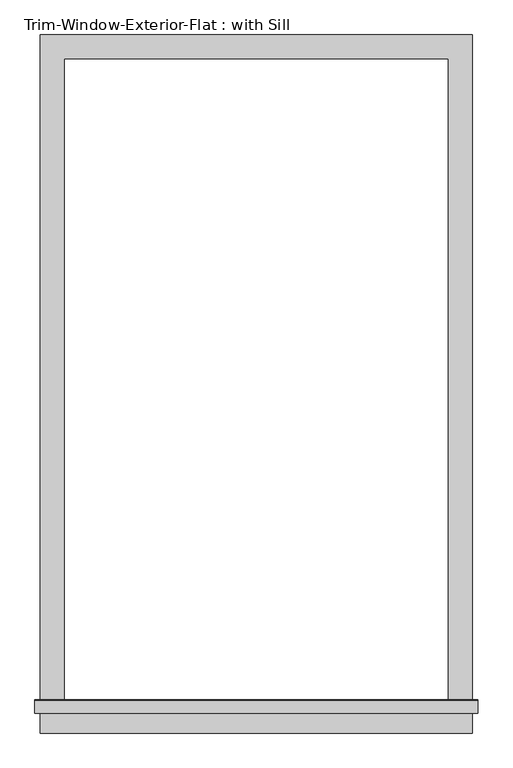
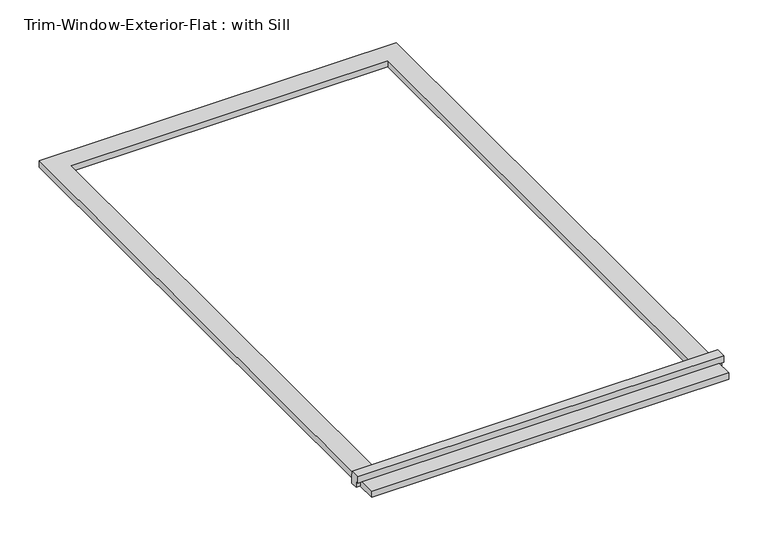
"""IFC4 building model written with IfcOpenShell, lengths in millimetres: proxy geometry, Trim-Window-Exterior-Flat : with Sill."""

import ifcopenshell
import ifcopenshell.guid

model = None  # the IFC model being written
_history = None  # IfcOwnerHistory: only IFC2X3 demands one
_inside = {}  # id of a spatial element -> (the spatial element, [elements in it])
_under = {}  # id of a project, library or spatial element -> (it, [spatial elements below it])
_declared = {}  # id of a project -> (the project, [libraries it declares])
_typed = {}  # id of a type object -> (the type object, [elements of that type])
_made_of = {}  # id of a material, layer set ... -> (it, [elements and type objects made of it])


def new_model(schema):
    """Start an empty IFC model of exactly this schema.

    Asked for "IFC4X3", IfcOpenShell would pick the latest addendum, in which some entities
    have other attributes; the version numbers below select the first issue.
    IFC2X3 requires an IfcOwnerHistory on every rooted entity: one is made here for all.
    """
    global model, _history
    if schema == "IFC4X3":
        model = ifcopenshell.file(schema_version=(4, 3, 0, 0))
    else:
        model = ifcopenshell.file(schema=schema)
    _inside.clear()
    _under.clear()
    _declared.clear()
    _typed.clear()
    _made_of.clear()
    _history = None
    if model.schema == "IFC2X3":
        org = make("IfcOrganization", Name="unknown")
        user = make(
            "IfcPersonAndOrganization",
            ThePerson=make("IfcPerson", FamilyName="unknown"),
            TheOrganization=org,
        )
        app = make(
            "IfcApplication",
            ApplicationDeveloper=org,
            Version="unknown",
            ApplicationFullName="unknown",
            ApplicationIdentifier="unknown",
        )
        _history = make(
            "IfcOwnerHistory",
            OwningUser=user,
            OwningApplication=app,
            ChangeAction="ADDED",
            CreationDate=0,
        )
    return model


def make(cls, **values):
    """One entity of the class cls with the attributes given. An attribute that is None is left unset."""
    return model.create_entity(
        cls, **{name: value for name, value in values.items() if value is not None}
    )


def rooted(cls, **values):
    """An entity with a GlobalId (a new one), such as an element, a storey or a relation."""
    return make(cls, GlobalId=ifcopenshell.guid.new(), OwnerHistory=_history, **values)


def si_unit(unit_type, name, prefix=None):
    """IfcSIUnit, for example si_unit("LENGTHUNIT", "METRE", prefix="MILLI")."""
    return make("IfcSIUnit", UnitType=unit_type, Prefix=prefix, Name=name)


def assignment(units):
    """IfcUnitAssignment: the units of a project."""
    return None if units is None else make("IfcUnitAssignment", Units=units)


def point(xyz):
    """IfcCartesianPoint."""
    return None if xyz is None else make("IfcCartesianPoint", Coordinates=xyz)


def direction(xyz):
    """IfcDirection."""
    return None if xyz is None else make("IfcDirection", DirectionRatios=xyz)


def frame(location, z_axis=None, x_axis=None):
    """IfcAxis2Placement3D, a coordinate frame: its origin and axes. An axis left out is left unset."""
    return make(
        "IfcAxis2Placement3D",
        Location=point(location),
        Axis=direction(z_axis),
        RefDirection=direction(x_axis),
    )


def origin():
    """The frame at (0, 0, 0) with its axes left unset."""
    return frame((0.0, 0.0, 0.0))


def origin_with_axes():
    """The frame at (0, 0, 0) with the z axis (0, 0, 1) and the x axis (1, 0, 0) written out."""
    return frame((0.0, 0.0, 0.0), z_axis=(0.0, 0.0, 1.0), x_axis=(1.0, 0.0, 0.0))


def place(relative_to, where):
    """IfcLocalPlacement: puts the frame where relative to a parent placement (None: the world)."""
    return make(
        "IfcLocalPlacement", PlacementRelTo=relative_to, RelativePlacement=where
    )


def context(
    kind, dimensions, precision=None, world=None, true_north=None, identifier=None
):
    """IfcGeometricRepresentationContext, for example the 3D "Model" context."""
    return make(
        "IfcGeometricRepresentationContext",
        ContextIdentifier=identifier,
        ContextType=kind,
        CoordinateSpaceDimension=dimensions,
        Precision=precision,
        WorldCoordinateSystem=world,
        TrueNorth=true_north,
    )


def project(units=None, contexts=None):
    """IfcProject with its units and contexts."""
    return rooted(
        "IfcProject",
        Name="project",
        RepresentationContexts=contexts,
        UnitsInContext=assignment(units),
    )


def spatial(cls, under=None, at=None, **own):
    """A site, building, storey or space (cls), placed at a placement, below another one or the project."""
    s = rooted(cls, ObjectPlacement=at, **own)
    if under is not None:
        _under.setdefault(under.id(), (under, []))[1].append(s)
    return s


def polyline(points):
    """IfcPolyline through the points."""
    return make("IfcPolyline", Points=[point(p) for p in points])


def outline(outer, holes=None, kind="AREA"):
    """IfcArbitraryClosedProfileDef: a profile drawn as a closed curve; with holes, ...WithVoids."""
    if holes is None:
        return make("IfcArbitraryClosedProfileDef", ProfileType=kind, OuterCurve=outer)
    return make(
        "IfcArbitraryProfileDefWithVoids",
        ProfileType=kind,
        OuterCurve=outer,
        InnerCurves=holes,
    )


def extrude(swept, where, along, depth):
    """IfcExtrudedAreaSolid: the profile swept, set in the frame where, extruded along a direction by depth."""
    return make(
        "IfcExtrudedAreaSolid",
        SweptArea=swept,
        Position=where,
        ExtrudedDirection=direction(along),
        Depth=depth,
    )


def shape(context_of_items, identifier, shape_type, items):
    """IfcShapeRepresentation: the items that make up one representation, for example the "Body"."""
    return make(
        "IfcShapeRepresentation",
        ContextOfItems=context_of_items,
        RepresentationIdentifier=identifier,
        RepresentationType=shape_type,
        Items=items,
    )


def source(mapping_origin, context_of_items, identifier, shape_type, items):
    """IfcRepresentationMap: a shape defined once, which mapped items show again and again."""
    return make(
        "IfcRepresentationMap",
        MappingOrigin=mapping_origin,
        MappedRepresentation=shape(context_of_items, identifier, shape_type, items),
    )


def transform(
    local_origin,
    x_axis=None,
    y_axis=None,
    z_axis=None,
    scale=None,
    scale2=None,
    scale3=None,
    uniform=True,
):
    """IfcCartesianTransformationOperator3D, or its non-uniform kind. x_axis, y_axis, z_axis: its Axis1, 2, 3."""
    if uniform:
        return make(
            "IfcCartesianTransformationOperator3D",
            Axis1=direction(x_axis),
            Axis2=direction(y_axis),
            LocalOrigin=point(local_origin),
            Scale=scale,
            Axis3=direction(z_axis),
        )
    return make(
        "IfcCartesianTransformationOperator3DnonUniform",
        Axis1=direction(x_axis),
        Axis2=direction(y_axis),
        LocalOrigin=point(local_origin),
        Scale=scale,
        Axis3=direction(z_axis),
        Scale2=scale2,
        Scale3=scale3,
    )


def mapped(mapping_source, mapping_target):
    """IfcMappedItem: shows the shape of a source again, moved by a transform."""
    return make(
        "IfcMappedItem", MappingSource=mapping_source, MappingTarget=mapping_target
    )


def made_of(thing, what):
    """Note that an element or type object is made of a material, layer set ...; save() writes the relation."""
    if what is not None:
        _made_of.setdefault(what.id(), (what, []))[1].append(thing)
    return thing


def element(
    cls,
    number,
    at=None,
    inside=None,
    cuts=None,
    type_object=None,
    material=None,
    context=None,
    identifier="Body",
    shape_type=None,
    held_by="IfcProductDefinitionShape",
    body=None,
    shapes=None,
    **own,
):
    """One element of the class cls, such as IfcWall. Its Tag is "e" and its number.

    at: its placement. inside: the storey or other place that contains it. cuts: it is an
    opening in that element (IfcRelVoidsElement). A single representation is given by context,
    identifier, shape_type and body (its items); several are given by shapes. held_by: the class
    of the entity that holds the representations. save() writes the other relations.
    """
    e = rooted(cls, Tag="e%d" % number, ObjectPlacement=at, **own)
    if body is not None:
        shapes = [shape(context, identifier, shape_type, body)]
    if shapes is not None:
        e.Representation = make(held_by, Representations=shapes)
    if inside is not None:
        _inside.setdefault(inside.id(), (inside, []))[1].append(e)
    if cuts is not None:
        rooted(
            "IfcRelVoidsElement", RelatingBuildingElement=cuts, RelatedOpeningElement=e
        )
    if type_object is not None:
        _typed.setdefault(type_object.id(), (type_object, []))[1].append(e)
    return made_of(e, material)


def aggregate(whole, parts):
    """IfcRelAggregates: a whole, such as a stair, and the parts it consists of."""
    return rooted("IfcRelAggregates", RelatingObject=whole, RelatedObjects=parts)


def save(model, path):
    """Write the relations noted so far, then the file.

    IfcRelAggregates (storeys below a building ...), IfcRelContainedInSpatialStructure (elements
    in a storey), IfcRelDefinesByType, IfcRelAssociatesMaterial and IfcRelDeclares: one each for
    every whole, place, type object, material and project.
    """
    for whole, parts in _under.values():
        aggregate(whole, parts)
    for where, things in _inside.values():
        rooted(
            "IfcRelContainedInSpatialStructure",
            RelatedElements=things,
            RelatingStructure=where,
        )
    for kind, things in _typed.values():
        rooted("IfcRelDefinesByType", RelatedObjects=things, RelatingType=kind)
    for what, things in _made_of.values():
        rooted("IfcRelAssociatesMaterial", RelatedObjects=things, RelatingMaterial=what)
    for by, libraries in _declared.values():
        rooted("IfcRelDeclares", RelatingContext=by, RelatedDefinitions=libraries)
    model.write(path)


def trim_window_exterior_flat_with_sill_48370fbd(model_context):
    return source(origin(), model_context, "Body", "SweptSolid", [
        extrude(outline(polyline([(514.35, -1546.1823709), (514.35, -1603.3323709), (-514.35, -1603.3323709), (-514.35, -1546.1823709), (514.35, -1546.1823709)])), origin_with_axes(), (0.0, 0.0, 1.0), 19.05),
        extrude(outline(polyline([(-1555.75, 38.1), (-1526.4580645, 38.1), (-1524.0, 19.05), (-1524.0, 0.0), (-1546.1823709, 0.0), (-1546.1823709, 19.05), (-1555.75, 19.05), (-1555.75, 38.1)])), frame((-527.05, 0.0, 0.0), z_axis=(1.0, 0.0, 0.0), x_axis=(0.0, 1.0, 0.0)), (0.0, 0.0, 1.0), 1054.1),
        extrude(outline(polyline([(-514.35, 57.15), (514.35, 57.15), (514.35, -1524.0), (457.2, -1524.0), (457.2, 0.0), (-457.2, 0.0), (-457.2, -1524.0), (-514.35, -1524.0), (-514.35, 57.15)])), origin_with_axes(), (0.0, 0.0, 1.0), 19.05),
    ])


if __name__ == "__main__":
    model = new_model("IFC4")
    model_context = context("Model", 3, world=origin())
    ifc_project = project(units=[si_unit("LENGTHUNIT", "METRE", prefix="MILLI")], contexts=[model_context])
    site = spatial("IfcSite", under=ifc_project)
    building = spatial("IfcBuilding", under=site)
    placement = place(None, origin())
    trim_window_exterior_flat_with_sill_shape = trim_window_exterior_flat_with_sill_48370fbd(model_context)
    element("IfcBuildingElementProxy", 1, Name="Trim-Window-Exterior-Flat : with Sill", ObjectType="Trim-Window-Exterior-Flat : with Sill", at=placement, inside=building, context=model_context, shape_type="MappedRepresentation", body=[
        mapped(trim_window_exterior_flat_with_sill_shape, transform((0.0, 0.0, 0.0), x_axis=(1.0, 0.0, 0.0), y_axis=(0.0, 1.0, 0.0), z_axis=(0.0, 0.0, 1.0))),
    ])
    save(model, "model.ifc")

# Revit data of these elements
# Type "Trim-Window-Exterior-Flat : with Sill"
#   Trim Width = 0' - 2 1/4"
#   Trim Thickness_Picture Frame = 0' - 1 1/4"
#   Trim Thickness_with Sill = 0' - 0 3/4"
#   Sill Thickness = 0' - 1 1/4"
#   Opening Width [instance default] = 2' - 0"
#   Opening Height [instance default] = 3' - 0"
#   Default Elevation = 4' - 0"
#   Sill = yes
#   Picture Frame = no
#   Trim Material [instance default] = none
# Element 1 (IfcBuildingElementProxy, "Trim-Window-Exterior-Flat : with Sill")
#   Opening Width = 3' - 0"
#   Opening Height = 5' - 0"
#   Trim Material = Clad - White
#   Materials on its faces: "Clad - White"
# Materials
#   "Clad - White": class "Wood", colour RGB 242 242 238, transparency 0, Cost = 0
